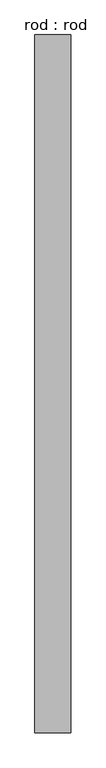
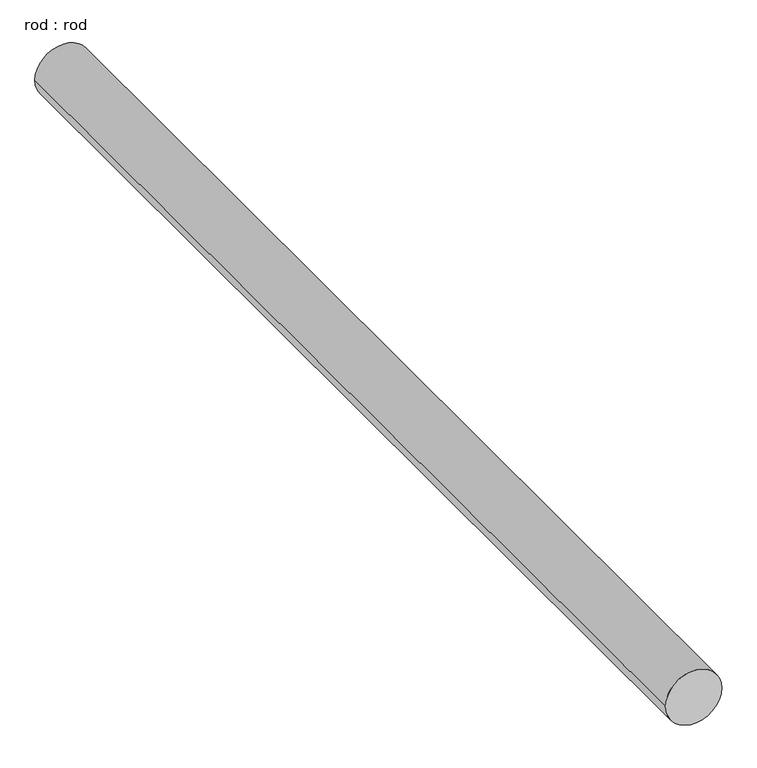
"""IFC4 building model written with IfcOpenShell, lengths in millimetres: proxy geometry, rod : rod."""

from ifc_helpers import new_model, si_unit, point, frame, frame_2d, origin, place, context, project, spatial, circle_curve, trimmed, segment, composite_curve, outline, extrude, source, transform, mapped, element, save


def rod_rod_a8841959(model_context):
    return source(origin(), model_context, "Body", "SweptSolid", [
        extrude(outline(composite_curve([segment(trimmed(circle_curve(frame_2d((0.0108462, 0.0)), 200.0), [point((0.0108462, 200.0))], [point((0.0108462, -200.0))], False, "CARTESIAN"), True, "CONTINUOUS"), segment(trimmed(circle_curve(frame_2d((0.0108462, 0.0)), 200.0), [point((0.0108462, -200.0))], [point((0.0108462, 200.0))], False, "CARTESIAN"), True, "CONTINUOUS")], self_intersect=False)), frame((0.0, 208.2434234, 0.0), z_axis=(0.0, 1.0, 0.0), x_axis=(0.0, 0.0, 1.0)), (0.0, 0.0, 1.0), 7768.9703839),
    ])


if __name__ == "__main__":
    model = new_model("IFC4")
    model_context = context("Model", 3, world=origin())
    ifc_project = project(units=[si_unit("LENGTHUNIT", "METRE", prefix="MILLI")], contexts=[model_context])
    site = spatial("IfcSite", under=ifc_project)
    building = spatial("IfcBuilding", under=site)
    placement = place(None, origin())
    rod_rod_shape = rod_rod_a8841959(model_context)
    element("IfcBuildingElementProxy", 1, Name="rod : rod", ObjectType="rod : rod", at=placement, inside=building, context=model_context, shape_type="MappedRepresentation", body=[
        mapped(rod_rod_shape, transform((0.0, 0.0, 0.0), x_axis=(1.0, 0.0, 0.0), y_axis=(0.0, 1.0, 0.0), z_axis=(0.0, 0.0, 1.0))),
    ])
    save(model, "model.ifc")

# Revit data of these elements
# Type "rod : rod"
#   Default Elevation = 0
